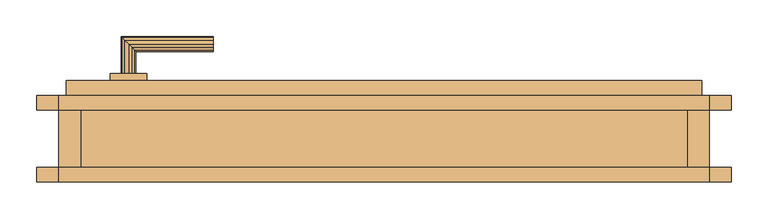
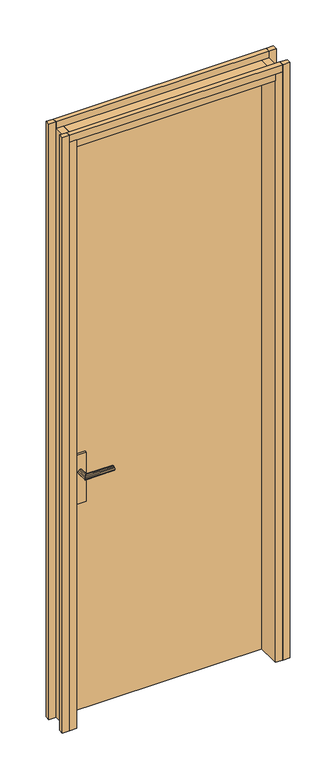
"""IFC4 building model written with IfcOpenShell, lengths in millimetres: door geometry, Tür."""

from ifc_helpers import new_model, si_unit, frame, origin, place, context, project, spatial, polyline, outline, extrude, faceted_brep, source, transform, mapped, element, save


def door_dc2b8873(model_context):
    return source(origin(), model_context, "Body", "SolidModel", [
        extrude(outline(polyline([(30.0, -20.0), (0.0, -20.0), (0.0, 98.0), (30.0, 98.0), (30.0, -20.0)])), frame((0.0, 0.0, 140.0), z_axis=(0.0, 0.0, 1.0), x_axis=(1.0, 0.0, 0.0)), (0.0, 0.0, 1.0), 2580.0),
        extrude(outline(polyline([(120.0, 118.0), (70.0, 118.0), (70.0, 128.0), (120.0, 128.0), (120.0, 118.0)])), frame((0.0, 0.0, 1050.0), z_axis=(0.0, 0.0, 1.0), x_axis=(1.0, 0.0, 0.0)), (0.0, 0.0, 1.0), 215.0),
        extrude(outline(polyline([(885.0, -20.0), (0.0, -20.0), (0.0, 0.0), (885.0, 0.0), (885.0, -20.0)])), frame((0.0, 0.0, 2720.0), z_axis=(0.0, 0.0, 1.0), x_axis=(1.0, 0.0, 0.0)), (0.0, 0.0, 1.0), 30.0),
        extrude(outline(polyline([(0.0, -20.0), (-30.0, -20.0), (-30.0, 0.0), (0.0, 0.0), (0.0, -20.0)])), frame((0.0, 0.0, 140.0), z_axis=(0.0, 0.0, 1.0), x_axis=(1.0, 0.0, 0.0)), (0.0, 0.0, 1.0), 2610.0),
        extrude(outline(polyline([(885.0, 78.0), (0.0, 78.0), (0.0, 98.0), (885.0, 98.0), (885.0, 78.0)])), frame((0.0, 0.0, 2720.0), z_axis=(0.0, 0.0, 1.0), x_axis=(1.0, 0.0, 0.0)), (0.0, 0.0, 1.0), 30.0),
        extrude(outline(polyline([(855.0, -20.0), (30.0, -20.0), (30.0, 98.0), (855.0, 98.0), (855.0, -20.0)])), frame((0.0, 0.0, 2690.0), z_axis=(0.0, 0.0, 1.0), x_axis=(1.0, 0.0, 0.0)), (0.0, 0.0, 1.0), 30.0),
        extrude(outline(polyline([(0.0, 78.0), (-30.0, 78.0), (-30.0, 98.0), (0.0, 98.0), (0.0, 78.0)])), frame((0.0, 0.0, 140.0), z_axis=(0.0, 0.0, 1.0), x_axis=(1.0, 0.0, 0.0)), (0.0, 0.0, 1.0), 2610.0),
        faceted_brep([(100.0, 128.0, 1198.660254), (95.0, 128.0, 1200.0), (90.0, 128.0, 1198.660254), (86.339746, 128.0, 1195.0), (85.0, 128.0, 1190.0), (86.339746, 128.0, 1185.0), (90.0, 128.0, 1181.339746), (95.0, 128.0, 1180.0), (100.0, 128.0, 1181.339746), (103.660254, 128.0, 1185.0), (105.0, 128.0, 1190.0), (103.660254, 128.0, 1195.0), (95.0, 168.0, 1200.0), (90.0, 173.0, 1198.660254), (86.339746, 176.660254, 1195.0), (85.0, 178.0, 1190.0), (86.339746, 176.660254, 1185.0), (90.0, 173.0, 1181.339746), (95.0, 168.0, 1180.0), (100.0, 163.0, 1181.339746), (103.660254, 159.339746, 1185.0), (105.0, 158.0, 1190.0), (103.660254, 159.339746, 1195.0), (100.0, 163.0, 1198.660254), (210.0, 173.0, 1198.660254), (210.0, 168.0, 1200.0), (210.0, 163.0, 1198.660254), (210.0, 159.339746, 1195.0), (210.0, 158.0, 1190.0), (210.0, 159.339746, 1185.0), (210.0, 163.0, 1181.339746), (210.0, 168.0, 1180.0), (210.0, 173.0, 1181.339746), (210.0, 176.660254, 1185.0), (210.0, 178.0, 1190.0), (210.0, 176.660254, 1195.0)], [[[0, 1, 2, 3, 4, 5, 6, 7, 8, 9, 10, 11]], [[2, 1, 12, 13]], [[3, 2, 13, 14]], [[4, 3, 14, 15]], [[5, 4, 15, 16]], [[6, 5, 16, 17]], [[7, 6, 17, 18]], [[8, 7, 18, 19]], [[9, 8, 19, 20]], [[10, 9, 20, 21]], [[11, 10, 21, 22]], [[0, 11, 22, 23]], [[1, 0, 23, 12]], [[24, 25, 26, 27, 28, 29, 30, 31, 32, 33, 34, 35]], [[13, 12, 25, 24]], [[14, 13, 24, 35]], [[15, 14, 35, 34]], [[16, 15, 34, 33]], [[17, 16, 33, 32]], [[18, 17, 32, 31]], [[19, 18, 31, 30]], [[20, 19, 30, 29]], [[21, 20, 29, 28]], [[22, 21, 28, 27]], [[23, 22, 27, 26]], [[12, 23, 26, 25]]]),
        extrude(outline(polyline([(70.0, 68.0), (70.0, 78.0), (120.0, 78.0), (120.0, 68.0), (70.0, 68.0)])), frame((0.0, 0.0, 1050.0), z_axis=(0.0, 0.0, 1.0), x_axis=(1.0, 0.0, 0.0)), (0.0, 0.0, 1.0), 215.0),
        extrude(outline(polyline([(885.0, -20.0), (855.0, -20.0), (855.0, 98.0), (885.0, 98.0), (885.0, -20.0)])), frame((0.0, 0.0, 140.0), z_axis=(0.0, 0.0, 1.0), x_axis=(1.0, 0.0, 0.0)), (0.0, 0.0, 1.0), 2580.0),
        extrude(outline(polyline([(915.0, 0.0), (915.0, -20.0), (885.0, -20.0), (885.0, 0.0), (915.0, 0.0)])), frame((0.0, 0.0, 140.0), z_axis=(0.0, 0.0, 1.0), x_axis=(1.0, 0.0, 0.0)), (0.0, 0.0, 1.0), 2610.0),
        extrude(outline(polyline([(875.0, 78.0), (10.0, 78.0), (10.0, 118.0), (875.0, 118.0), (875.0, 78.0)])), frame((0.0, 0.0, 140.0), z_axis=(0.0, 0.0, 1.0), x_axis=(1.0, 0.0, 0.0)), (0.0, 0.0, 1.0), 2570.0),
        extrude(outline(polyline([(915.0, 98.0), (915.0, 78.0), (885.0, 78.0), (885.0, 98.0), (915.0, 98.0)])), frame((0.0, 0.0, 140.0), z_axis=(0.0, 0.0, 1.0), x_axis=(1.0, 0.0, 0.0)), (0.0, 0.0, 1.0), 2610.0),
        faceted_brep([(90.0, 68.0, 1198.660254), (95.0, 68.0, 1200.0), (100.0, 68.0, 1198.660254), (103.660254, 68.0, 1195.0), (105.0, 68.0, 1190.0), (103.660254, 68.0, 1185.0), (100.0, 68.0, 1181.339746), (95.0, 68.0, 1180.0), (90.0, 68.0, 1181.339746), (86.339746, 68.0, 1185.0), (85.0, 68.0, 1190.0), (86.339746, 68.0, 1195.0), (95.0, 28.0, 1200.0), (90.0, 23.0, 1198.660254), (86.339746, 19.339746, 1195.0), (85.0, 18.0, 1190.0), (86.339746, 19.339746, 1185.0), (90.0, 23.0, 1181.339746), (95.0, 28.0, 1180.0), (100.0, 33.0, 1181.339746), (103.660254, 36.660254, 1185.0), (105.0, 38.0, 1190.0), (103.660254, 36.660254, 1195.0), (100.0, 33.0, 1198.660254), (210.0, 33.0, 1198.660254), (210.0, 28.0, 1200.0), (210.0, 23.0, 1198.660254), (210.0, 19.339746, 1195.0), (210.0, 18.0, 1190.0), (210.0, 19.339746, 1185.0), (210.0, 23.0, 1181.339746), (210.0, 28.0, 1180.0), (210.0, 33.0, 1181.339746), (210.0, 36.660254, 1185.0), (210.0, 38.0, 1190.0), (210.0, 36.660254, 1195.0)], [[[0, 1, 2, 3, 4, 5, 6, 7, 8, 9, 10, 11]], [[12, 1, 0, 13]], [[13, 0, 11, 14]], [[14, 11, 10, 15]], [[15, 10, 9, 16]], [[16, 9, 8, 17]], [[17, 8, 7, 18]], [[18, 7, 6, 19]], [[19, 6, 5, 20]], [[20, 5, 4, 21]], [[21, 4, 3, 22]], [[22, 3, 2, 23]], [[23, 2, 1, 12]], [[24, 25, 26, 27, 28, 29, 30, 31, 32, 33, 34, 35]], [[25, 12, 13, 26]], [[26, 13, 14, 27]], [[27, 14, 15, 28]], [[28, 15, 16, 29]], [[29, 16, 17, 30]], [[30, 17, 18, 31]], [[31, 18, 19, 32]], [[32, 19, 20, 33]], [[33, 20, 21, 34]], [[34, 21, 22, 35]], [[35, 22, 23, 24]], [[24, 23, 12, 25]]]),
    ])


if __name__ == "__main__":
    model = new_model("IFC4")
    model_context = context("Model", 3, world=origin())
    ifc_project = project(units=[si_unit("LENGTHUNIT", "METRE", prefix="MILLI")], contexts=[model_context])
    site = spatial("IfcSite", under=ifc_project)
    building = spatial("IfcBuilding", under=site)
    placement = place(None, origin())
    door_shape = door_dc2b8873(model_context)
    element("IfcDoor", 1, ObjectType="Tür", at=placement, inside=building, context=model_context, shape_type="MappedRepresentation", body=[
        mapped(door_shape, transform((0.0, 0.0, 0.0), x_axis=(1.0, 0.0, 0.0), y_axis=(0.0, 1.0, 0.0), z_axis=(0.0, 0.0, 1.0))),
    ])
    save(model, "model.ifc")

# Revit data of these elements
# Type "Tür"
#   Type Mark = "50"
# Element 1 (IfcDoor, "Tür")
#   Materials on its faces: "tuer_beschlag", "tuer_holzzarge"
# Materials
#   "tuer_beschlag": class "Unassigned", colour RGB 128 128 128, transparency 0
#   "tuer_holzzarge": class "Unassigned", colour RGB 255 255 255, transparency 0
